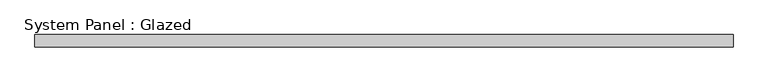
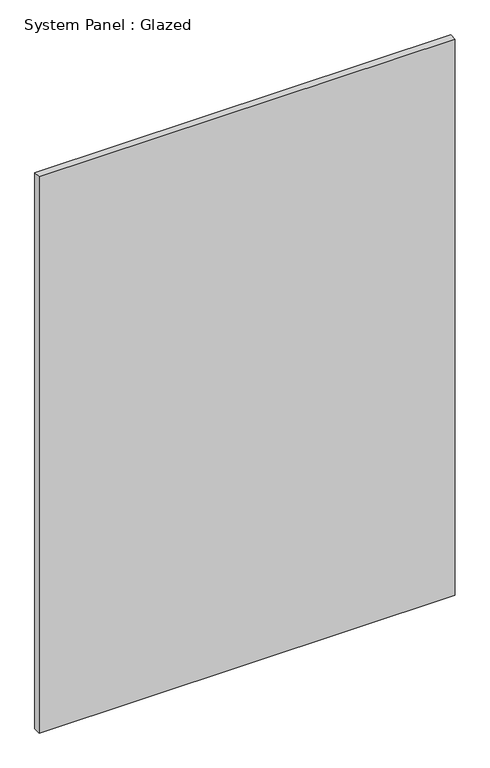
"""IFC4 building model written with IfcOpenShell, lengths in millimetres: plate geometry, System Panel : Glazed."""

from ifc_helpers import new_model, si_unit, origin, origin_with_axes, place, context, project, spatial, polyline, outline, extrude, source, transform, mapped, element, save


def system_panel_glazed_af99cf8b(model_context):
    return source(origin(), model_context, "Body", "SweptSolid", [
        extrude(outline(polyline([(719.3802866, 19.05), (-719.3802866, 19.05), (-719.3802866, 44.45), (719.3802866, 44.45), (719.3802866, 19.05)])), origin_with_axes(), (0.0, 0.0, 1.0), 2032.8912782),
    ])


if __name__ == "__main__":
    model = new_model("IFC4")
    model_context = context("Model", 3, world=origin())
    ifc_project = project(units=[si_unit("LENGTHUNIT", "METRE", prefix="MILLI")], contexts=[model_context])
    site = spatial("IfcSite", under=ifc_project)
    building = spatial("IfcBuilding", under=site)
    placement = place(None, origin())
    system_panel_glazed_shape = system_panel_glazed_af99cf8b(model_context)
    element("IfcPlate", 1, ObjectType="System Panel : Glazed", at=placement, inside=building, context=model_context, shape_type="MappedRepresentation", body=[
        mapped(system_panel_glazed_shape, transform((0.0, 0.0, 0.0), x_axis=(1.0, 0.0, 0.0), y_axis=(0.0, 1.0, 0.0), z_axis=(0.0, 0.0, 1.0))),
    ])
    save(model, "model.ifc")

# Revit data of these elements
# Type "System Panel : Glazed"
#   Construction Type Id = "GSP4R"
#   Analytic Construction = "1/8 in Pilkington single glazing"
#   Visual Light Transmittance = 0.9
#   Solar Heat Gain Coefficient = 0.86
#   Heat Transfer Coefficient (U) = 1.18115 BTU/(h·ft²·°F)
#   Define Thermal Properties by = 1
# Element 1 (IfcPlate, "System Panel : Glazed")
#   Materials on its faces: "Glass"
# Materials
#   "Glass": class "Glass", colour RGB 0 128 192, transparency 0.75, Description = "Soda Lime Glass", Cost = 0
